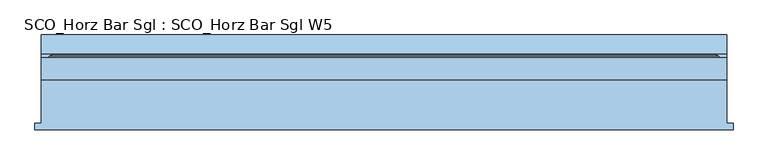
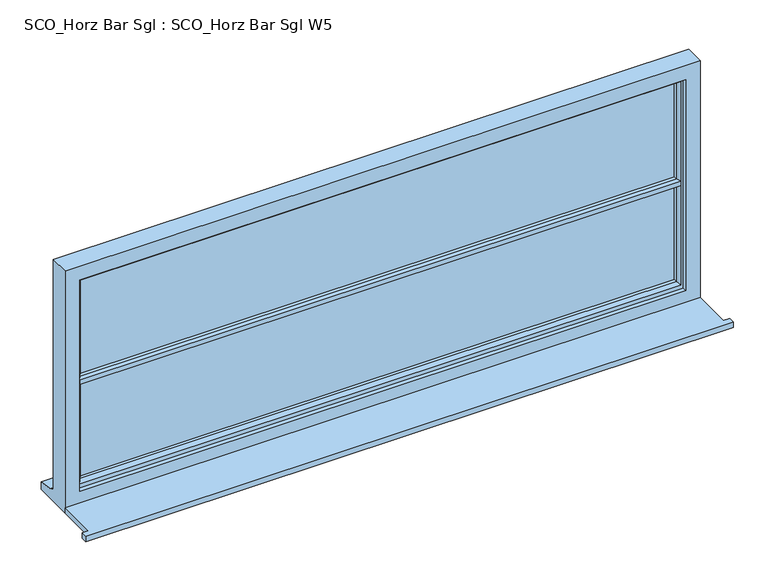
"""IFC4 building model written with IfcOpenShell, lengths in millimetres: window geometry, SCO_Horz Bar Sgl : SCO_Horz Bar Sgl W5."""

from ifc_helpers import new_model, si_unit, frame, origin, place, context, project, spatial, polyline, outline, extrude, faceted_brep, source, transform, mapped, element, save


def sco_horz_bar_sgl_sco_horz_bar_sgl_w5_3eb3dd01(model_context):
    return source(origin(), model_context, "Body", "SolidModel", [
        extrude(outline(polyline([(-1325.0, -191.5434322), (-1325.0, -166.5434322), (-1300.0, -166.5434322), (-1300.0, -2.0434322), (1300.0, -2.0434322), (1300.0, -166.5434322), (1325.0, -166.5434322), (1325.0, -191.5434322), (-1325.0, -191.5434322)])), frame((0.0, 0.0, 1060.0), z_axis=(0.0, 0.0, 1.0), x_axis=(1.0, 0.0, 0.0)), (0.0, 0.0, 1.0), 25.0),
        faceted_brep([(-1300.0, -2.0434322, 1060.0), (1300.0, -2.0434322, 1060.0), (1300.0, -2.0434322, 2110.0), (-1300.0, -2.0434322, 2110.0), (-1240.0, -2.0434322, 2050.0), (1240.0, -2.0434322, 2050.0), (1240.0, -2.0434322, 1135.0), (-1240.0, -2.0434322, 1135.0), (-1300.0, 80.9565678, 2110.0), (-1300.0, 80.9565678, 1111.0), (-1300.0, 95.9565678, 1109.68767), (-1300.0, 95.9565678, 1104.7449676), (-1300.0, 168.4565678, 1093.8088847), (-1300.0, 168.4565678, 1060.0), (1300.0, 80.9565678, 2110.0), (1300.0, 80.9565678, 1111.0), (-1260.0, 80.9565678, 2070.0), (-1260.0, 80.9565678, 1123.0), (1260.0, 80.9565678, 1123.0), (1260.0, 80.9565678, 2070.0), (-1260.0, 15.9565678, 2070.0), (-1260.0, 15.9565678, 1123.0), (1260.0, 15.9565678, 2070.0), (1260.0, 15.9565678, 1123.0), (-1240.0, 15.9565678, 2050.0), (-1240.0, 15.9565678, 1135.0), (1240.0, 15.9565678, 1135.0), (1240.0, 15.9565678, 2050.0), (1300.0, 168.4565678, 1060.0), (1300.0, 168.4565678, 1093.8088847), (1300.0, 95.9565678, 1104.7449676), (1300.0, 95.9565678, 1109.68767)], [[[0, 1, 2, 3], [4, 5, 6, 7]], [[0, 3, 8, 9, 10, 11, 12, 13]], [[9, 8, 14, 15], [16, 17, 18, 19]], [[17, 16, 20, 21]], [[20, 22, 23, 21], [24, 25, 26, 27]], [[24, 4, 7, 25]], [[3, 2, 14, 8]], [[16, 19, 22, 20]], [[5, 4, 24, 27]], [[15, 14, 2, 1, 28, 29, 30, 31]], [[19, 18, 23, 22]], [[5, 27, 26, 6]], [[28, 1, 0, 13]], [[29, 28, 13, 12]], [[30, 29, 12, 11]], [[31, 30, 11, 10]], [[15, 31, 10, 9]], [[21, 23, 18, 17]], [[7, 6, 26, 25]]]),
        extrude(outline(polyline([(1230.1480377, 44.9565678), (-1230.0, 44.9565678), (-1230.0, 68.9565678), (1230.1480377, 68.9565678), (1230.1480377, 44.9565678)])), frame((0.0, 0.0, 1153.0), z_axis=(0.0, 0.0, 1.0), x_axis=(1.0, 0.0, 0.0)), (0.0, 0.0, 1.0), 434.3307627),
        extrude(outline(polyline([(1230.1480377, 44.9565678), (-1230.0, 44.9565678), (-1230.0, 68.9565678), (1230.1480377, 68.9565678), (1230.1480377, 44.9565678)])), frame((0.0, 0.0, 1597.6692373), z_axis=(0.0, 0.0, 1.0), x_axis=(1.0, 0.0, 0.0)), (0.0, 0.0, 1.0), 442.3307627),
        extrude(outline(polyline([(92.5035732, 1597.6692373), (92.5035732, 1587.3307627), (86.8277797, 1577.5), (68.9565678, 1577.5), (68.9565678, 1584.5), (44.9565678, 1584.5), (44.9565678, 1577.5), (30.4494677, 1577.5), (15.9565678, 1582.6480377), (15.9565678, 1602.3519623), (30.4494677, 1607.5), (44.9565678, 1607.5), (44.9565678, 1600.5), (68.9565678, 1600.5), (68.9565678, 1607.5), (86.8277797, 1607.5), (92.5035732, 1597.6692373)])), frame((-1230.1480377, 0.0, 0.0), z_axis=(1.0, 0.0, 0.0), x_axis=(0.0, 1.0, 0.0)), (0.0, 0.0, 1.0), 2460.2960754),
        faceted_brep([(-1270.0, 80.9565678, 2072.0), (-1270.0, 86.7300705, 2072.0), (-1270.0, 86.7300705, 1113.0), (-1270.0, 80.9565678, 1113.0), (-1260.0, 15.9565678, 2062.0), (-1260.0, 80.9565678, 2062.0), (-1260.0, 80.9565678, 1123.0), (-1260.0, 15.9565678, 1123.0), (-1220.0, 30.4494677, 2022.0), (-1230.1480377, 15.9565678, 2032.1480377), (-1230.1480377, 15.9565678, 1152.8519623), (-1220.0, 30.4494677, 1163.0), (-1220.0, 44.9565678, 2022.0), (-1220.0, 44.9565678, 1163.0), (-1230.0, 68.9565678, 2032.0), (-1230.0, 44.9565678, 2032.0), (-1230.0, 44.9565678, 1153.0), (-1230.0, 68.9565678, 1153.0), (-1220.0, 86.7300705, 2022.0), (-1220.0, 68.9565678, 2022.0), (-1220.0, 68.9565678, 1163.0), (-1220.0, 86.7300705, 1163.0), (-1230.0, 92.5035732, 2032.0), (-1230.0, 92.5035732, 1153.0), (-1259.2153903, 92.5035732, 2061.2153903), (-1259.2153903, 92.5035732, 1123.7846097), (1270.0, 86.7300705, 1113.0), (1270.0, 80.9565678, 1113.0), (1260.0, 80.9565678, 1123.0), (1260.0, 15.9565678, 1123.0), (1230.1480377, 15.9565678, 1152.8519623), (1220.0, 30.4494677, 1163.0), (1220.0, 44.9565678, 1163.0), (1230.0, 44.9565678, 1153.0), (1230.0, 68.9565678, 1153.0), (1220.0, 68.9565678, 1163.0), (1220.0, 86.7300705, 1163.0), (1230.0, 92.5035732, 1153.0), (1259.2153903, 92.5035732, 1123.7846097), (1270.0, 86.7300705, 2072.0), (1270.0, 80.9565678, 2072.0), (1260.0, 80.9565678, 2062.0), (1260.0, 15.9565678, 2062.0), (1230.1480377, 15.9565678, 2032.1480377), (1220.0, 30.4494677, 2022.0), (1220.0, 44.9565678, 2022.0), (1230.0, 44.9565678, 2032.0), (1230.0, 68.9565678, 2032.0), (1220.0, 68.9565678, 2022.0), (1220.0, 86.7300705, 2022.0), (1230.0, 92.5035732, 2032.0), (1259.2153903, 92.5035732, 2061.2153903)], [[[0, 1, 2, 3]], [[4, 5, 6, 7]], [[8, 9, 10, 11]], [[12, 8, 11, 13]], [[14, 15, 16, 17]], [[18, 19, 20, 21]], [[22, 18, 21, 23]], [[1, 24, 25, 2]], [[3, 2, 26, 27]], [[7, 6, 28, 29]], [[11, 10, 30, 31]], [[13, 11, 31, 32]], [[17, 16, 33, 34]], [[21, 20, 35, 36]], [[23, 21, 36, 37]], [[2, 25, 38, 26]], [[27, 26, 39, 40]], [[29, 28, 41, 42]], [[31, 30, 43, 44]], [[32, 31, 44, 45]], [[34, 33, 46, 47]], [[36, 35, 48, 49]], [[37, 36, 49, 50]], [[26, 38, 51, 39]], [[40, 39, 1, 0]], [[3, 27, 40, 0], [5, 41, 28, 6]], [[42, 41, 5, 4]], [[7, 29, 42, 4], [9, 43, 30, 10]], [[44, 43, 9, 8]], [[45, 44, 8, 12]], [[15, 46, 33, 16], [13, 32, 45, 12]], [[47, 46, 15, 14]], [[17, 34, 47, 14], [19, 48, 35, 20]], [[49, 48, 19, 18]], [[50, 49, 18, 22]], [[24, 51, 38, 25], [23, 37, 50, 22]], [[39, 51, 24, 1]]]),
    ])


if __name__ == "__main__":
    model = new_model("IFC4")
    model_context = context("Model", 3, world=origin())
    ifc_project = project(units=[si_unit("LENGTHUNIT", "METRE", prefix="MILLI")], contexts=[model_context])
    site = spatial("IfcSite", under=ifc_project)
    building = spatial("IfcBuilding", under=site)
    placement = place(None, origin())
    sco_horz_bar_sgl_sco_horz_bar_sgl_w5_shape = sco_horz_bar_sgl_sco_horz_bar_sgl_w5_3eb3dd01(model_context)
    element("IfcWindow", 1, ObjectType="SCO_Horz Bar Sgl : SCO_Horz Bar Sgl W5", at=placement, inside=building, context=model_context, shape_type="MappedRepresentation", body=[
        mapped(sco_horz_bar_sgl_sco_horz_bar_sgl_w5_shape, transform((0.0, 0.0, 0.0), x_axis=(1.0, 0.0, 0.0), y_axis=(0.0, 1.0, 0.0), z_axis=(0.0, 0.0, 1.0))),
    ])
    save(model, "model.ifc")

# Revit data of these elements
# Type "SCO_Horz Bar Sgl : SCO_Horz Bar Sgl W5"
#   Type Mark = "W5"
#   Operation = "SinglePanel"
#   Manufacturer = "Revit"
#   Keynote = "L10"
#   Wrap Layers (Ext) from Ext = 102.5 mm
#   Wrap Layers (Int) from Ext = 177.5 mm
#   Window Board Projection = 25 mm
#   Window Board Extension = 25 mm
#   Rough Width = 2600 mm
#   Rough Height = 1050 mm
#   Height = 1050 mm
#   Width = 2600 mm
#   Glazing Thickness = 24 mm
#   FrameOffset - External = 102.5 mm
#   Frame Depth = 65 mm
#   Ext Leaf Thickness (Scot) = 102.5 mm
#   Ext Leaf Overlap (Scot) = 25 mm
#   Default Head Height = 2110 mm
#   Cill Depth = 87.5 mm
#   Cavity Closer Width = 50 mm
#   Cavity Closer Offset from Ext = 102.5 mm
#   Cavity Closer Depth = 85 mm
#   Vis - Cavity Closers = yes
#   Material Trim = Window Frame
#   Material Glass = Glass
#   Material Frame = Window Frame
#   Wall Closure = (empty or 0)
# Element 1 (IfcWindow, "SCO_Horz Bar Sgl : SCO_Horz Bar Sgl W5")
#   Materials on its faces: "Window Frame", "Glass"
# Materials
#   "Window Frame": class "Miscellaneous", colour RGB 249 249 249, transparency 0
#   "Glass": class "Glass", colour RGB 0 128 192, transparency 0.75
